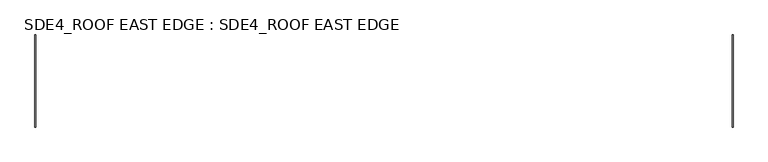
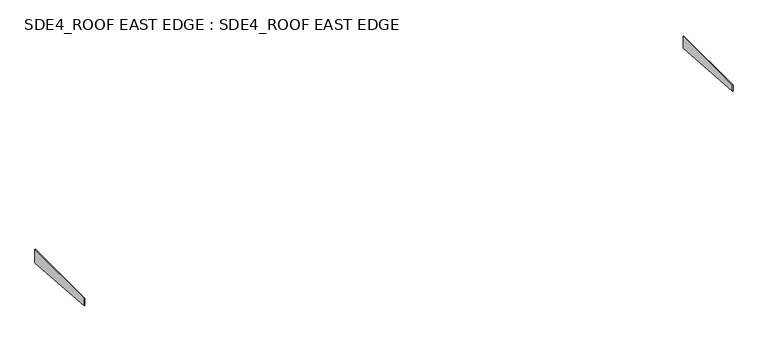
"""IFC4 building model written with IfcOpenShell, lengths in millimetres: proxy geometry, SDE4_ROOF EAST EDGE : SDE4_ROOF EAST EDGE."""

from ifc_helpers import new_model, si_unit, frame, origin, place, context, project, spatial, polyline, outline, extrude, source, transform, mapped, element, save


def sde4_roof_east_edge_sde4_roof_east_edge_7e08855c(model_context):
    return source(origin(), model_context, "Body", "SweptSolid", [
        extrude(outline(polyline([(-8295.0, 150096.6702289), (1900.0, 150096.6702289), (1900.0, 148414.6819707), (-8295.0, 149195.9937751), (-8295.0, 150096.6702289)])), frame((-324.5990437, 0.0, 0.0), z_axis=(1.0, 0.0, 0.0), x_axis=(0.0, 1.0, 0.0)), (0.0, 0.0, 1.0), 75.0),
        extrude(outline(polyline([(-8295.0, 149946.6702289), (1900.0, 149946.6702289), (1900.0, 148414.6819707), (-8295.0, 149195.9937751), (-8295.0, 149946.6702289)])), frame((76850.0, 0.0, 0.0), z_axis=(1.0, 0.0, 0.0), x_axis=(0.0, 1.0, 0.0)), (0.0, 0.0, 1.0), 75.0),
    ])


if __name__ == "__main__":
    model = new_model("IFC4")
    model_context = context("Model", 3, world=origin())
    ifc_project = project(units=[si_unit("LENGTHUNIT", "METRE", prefix="MILLI")], contexts=[model_context])
    site = spatial("IfcSite", under=ifc_project)
    building = spatial("IfcBuilding", under=site)
    placement = place(None, origin())
    sde4_roof_east_edge_sde4_roof_east_edge_shape = sde4_roof_east_edge_sde4_roof_east_edge_7e08855c(model_context)
    element("IfcBuildingElementProxy", 1, Name="SDE4_ROOF EAST EDGE : SDE4_ROOF EAST EDGE", ObjectType="SDE4_ROOF EAST EDGE : SDE4_ROOF EAST EDGE", at=placement, inside=building, context=model_context, shape_type="MappedRepresentation", body=[
        mapped(sde4_roof_east_edge_sde4_roof_east_edge_shape, transform((0.0, 0.0, 0.0), x_axis=(1.0, 0.0, 0.0), y_axis=(0.0, 1.0, 0.0), z_axis=(0.0, 0.0, 1.0))),
    ])
    save(model, "model.ifc")
